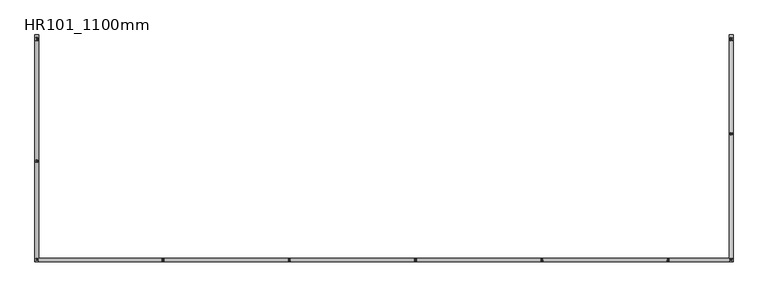
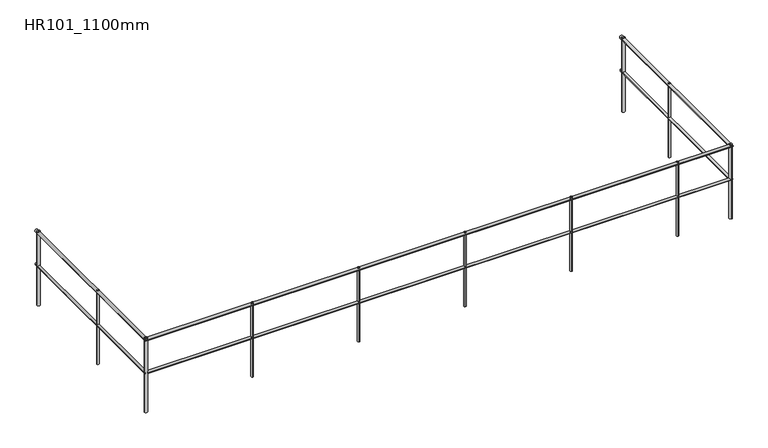
"""IFC4 building model written with IfcOpenShell, lengths in millimetres: railing geometry, HR101_1100mm."""

from ifc_helpers import new_model, si_unit, point, frame, frame_2d, origin, place, context, project, spatial, circle_curve, ellipse_curve, trimmed, segment, composite_curve, outline, extrude, source, transform, mapped, element, save
from ifc_brep_helpers import plane_surface, cylinder_surface, advanced_brep


def hr101_1100mm_fbcf2329(model_context):
    return source(origin(), model_context, "Body", "SolidModel", [
        advanced_brep(
        [(3942.0, 20699.5208589, 10633.005241), (3908.0, 20699.5208589, 10633.005241), (3942.0, 18041.5208589, 10633.005241), (3908.0, 18007.5208589, 10633.005241), (12158.0, 18041.5208589, 10633.005241), (12192.0, 18007.5208589, 10633.005241), (12158.0, 20699.5208589, 10633.005241), (12192.0, 20699.5208589, 10633.005241)],
        [
            (0, 1, circle_curve(frame((3925.0, 20699.5208589, 10633.005241), z_axis=(0.0, 1.0, 0.0), x_axis=(-1.0, 0.0, 0.0)), 17.0)),
            (1, 0, circle_curve(frame((3925.0, 20699.5208589, 10633.005241), z_axis=(0.0, 1.0, 0.0), x_axis=(-1.0, 0.0, 0.0)), 17.0)),
            (0, 2),
            (2, 3, ellipse_curve(frame((3925.0, 18024.5208589, 10633.005241), z_axis=(-0.7071067811865475, 0.7071067811865475, 0.0), x_axis=(0.7071067811865474, 0.7071067811865476, 0.0)), 24.0416306, 17.0)),
            (3, 1),
            (3, 2, ellipse_curve(frame((3925.0, 18024.5208589, 10633.005241), z_axis=(-0.7071067811865475, 0.7071067811865475, 0.0), x_axis=(0.7071067811865474, 0.7071067811865476, 0.0)), 24.0416306, 17.0)),
            (2, 4),
            (4, 5, ellipse_curve(frame((12175.0, 18024.5208589, 10633.005241), z_axis=(-0.7071067811865475, -0.7071067811865475, 0.0), x_axis=(-0.7071067811865476, 0.7071067811865474, 0.0)), 24.0416306, 17.0)),
            (5, 3),
            (5, 4, ellipse_curve(frame((12175.0, 18024.5208589, 10633.005241), z_axis=(-0.7071067811865475, -0.7071067811865475, 0.0), x_axis=(-0.7071067811865476, 0.7071067811865474, 0.0)), 24.0416306, 17.0)),
            (6, 7, circle_curve(frame((12175.0, 20699.5208589, 10633.005241), z_axis=(0.0, 1.0, 0.0), x_axis=(1.0, 0.0, 0.0)), 17.0)),
            (7, 6, circle_curve(frame((12175.0, 20699.5208589, 10633.005241), z_axis=(0.0, 1.0, 0.0), x_axis=(1.0, 0.0, 0.0)), 17.0)),
            (4, 6),
            (7, 5),
        ],
        [
            plane_surface(frame((3925.0, 20699.5208589, 10650.005241), z_axis=(0.0, 1.0, 0.0), x_axis=(0.0, 0.0, -1.0))),
            cylinder_surface(frame((3925.0, 20699.5208589, 10633.005241), z_axis=(0.0, 1.0, 0.0), x_axis=(-1.0, 0.0, 0.0)), 17.0),
            cylinder_surface(frame((3925.0, 18024.5208589, 10633.005241), z_axis=(-1.0, 0.0, 0.0), x_axis=(0.0, -1.0, 0.0)), 17.0),
            plane_surface(frame((12175.0, 20699.5208589, 10650.005241), z_axis=(0.0, 1.0, 0.0), x_axis=(0.0, 0.0, 1.0))),
            cylinder_surface(frame((12175.0, 18024.5208589, 10633.005241), z_axis=(0.0, -1.0, 0.0), x_axis=(1.0, 0.0, 0.0)), 17.0),
        ],
        [
            (0, [[1, 2]]),
            (1, [[-1, 3, 4, 5]]),
            (1, [[-2, -5, 6, -3]]),
            (2, [[-4, 7, 8, 9]]),
            (2, [[-6, -9, 10, -7]]),
            (3, [[11, 12]]),
            (4, [[-8, 13, -12, 14]]),
            (4, [[-10, -14, -11, -13]]),
        ],
    ),
        advanced_brep(
        [(3946.35, 20699.5208589, 11128.655241), (3903.65, 20699.5208589, 11128.655241), (3946.35, 18045.8708589, 11128.655241), (3903.65, 18003.1708589, 11128.655241), (12153.65, 18045.8708589, 11128.655241), (12196.35, 18003.1708589, 11128.655241), (12153.65, 20699.5208589, 11128.655241), (12196.35, 20699.5208589, 11128.655241)],
        [
            (0, 1, circle_curve(frame((3925.0, 20699.5208589, 11128.655241), z_axis=(0.0, 1.0, 0.0), x_axis=(-1.0, 0.0, 0.0)), 21.35)),
            (1, 0, circle_curve(frame((3925.0, 20699.5208589, 11128.655241), z_axis=(0.0, 1.0, 0.0), x_axis=(-1.0, 0.0, 0.0)), 21.35)),
            (0, 2),
            (2, 3, ellipse_curve(frame((3925.0, 18024.5208589, 11128.655241), z_axis=(-0.7071067811865475, 0.7071067811865475, 0.0), x_axis=(0.7071067811865474, 0.7071067811865476, 0.0)), 30.1934596, 21.35)),
            (3, 1),
            (3, 2, ellipse_curve(frame((3925.0, 18024.5208589, 11128.655241), z_axis=(-0.7071067811865475, 0.7071067811865475, 0.0), x_axis=(0.7071067811865474, 0.7071067811865476, 0.0)), 30.1934596, 21.35)),
            (2, 4),
            (4, 5, ellipse_curve(frame((12175.0, 18024.5208589, 11128.655241), z_axis=(-0.7071067811865475, -0.7071067811865475, 0.0), x_axis=(-0.7071067811865476, 0.7071067811865474, 0.0)), 30.1934596, 21.35)),
            (5, 3),
            (5, 4, ellipse_curve(frame((12175.0, 18024.5208589, 11128.655241), z_axis=(-0.7071067811865475, -0.7071067811865475, 0.0), x_axis=(-0.7071067811865476, 0.7071067811865474, 0.0)), 30.1934596, 21.35)),
            (6, 7, circle_curve(frame((12175.0, 20699.5208589, 11128.655241), z_axis=(0.0, 1.0, 0.0), x_axis=(1.0, 0.0, 0.0)), 21.35)),
            (7, 6, circle_curve(frame((12175.0, 20699.5208589, 11128.655241), z_axis=(0.0, 1.0, 0.0), x_axis=(1.0, 0.0, 0.0)), 21.35)),
            (4, 6),
            (7, 5),
        ],
        [
            plane_surface(frame((3925.0, 20699.5208589, 11150.005241), z_axis=(0.0, 1.0, 0.0), x_axis=(0.0, 0.0, -1.0))),
            cylinder_surface(frame((3925.0, 20699.5208589, 11128.655241), z_axis=(0.0, 1.0, 0.0), x_axis=(-1.0, 0.0, 0.0)), 21.35),
            cylinder_surface(frame((3925.0, 18024.5208589, 11128.655241), z_axis=(-1.0, 0.0, 0.0), x_axis=(0.0, -1.0, 0.0)), 21.35),
            plane_surface(frame((12175.0, 20699.5208589, 11150.005241), z_axis=(0.0, 1.0, 0.0), x_axis=(0.0, 0.0, 1.0))),
            cylinder_surface(frame((12175.0, 18024.5208589, 11128.655241), z_axis=(0.0, -1.0, 0.0), x_axis=(1.0, 0.0, 0.0)), 21.35),
        ],
        [
            (0, [[1, 2]]),
            (1, [[-1, 3, 4, 5]]),
            (1, [[-2, -5, 6, -3]]),
            (2, [[-4, 7, 8, 9]]),
            (2, [[-6, -9, 10, -7]]),
            (3, [[11, 12]]),
            (4, [[-8, 13, -12, 14]]),
            (4, [[-10, -14, -11, -13]]),
        ],
    ),
        extrude(outline(composite_curve([segment(trimmed(circle_curve(frame_2d((12175.0, 19524.5208589)), 15.0), [point((12190.0, 19524.5208589))], [point((12160.0, 19524.5208589))], False, "CARTESIAN"), True, "CONTINUOUS"), segment(trimmed(circle_curve(frame_2d((12175.0, 19524.5208589)), 15.0), [point((12160.0, 19524.5208589))], [point((12190.0, 19524.5208589))], False, "CARTESIAN"), True, "CONTINUOUS")], self_intersect=False)), frame((0.0, 0.0, 10050.005241), z_axis=(0.0, 0.0, 1.0), x_axis=(1.0, 0.0, 0.0)), (0.0, 0.0, 1.0), 1100.0),
        extrude(outline(composite_curve([segment(trimmed(circle_curve(frame_2d((11425.0, 18024.5208589)), 15.0), [point((11425.0, 18009.5208589))], [point((11425.0, 18039.5208589))], False, "CARTESIAN"), True, "CONTINUOUS"), segment(trimmed(circle_curve(frame_2d((11425.0, 18024.5208589)), 15.0), [point((11425.0, 18039.5208589))], [point((11425.0, 18009.5208589))], False, "CARTESIAN"), True, "CONTINUOUS")], self_intersect=False)), frame((0.0, 0.0, 10050.005241), z_axis=(0.0, 0.0, 1.0), x_axis=(1.0, 0.0, 0.0)), (0.0, 0.0, 1.0), 1100.0),
        extrude(outline(composite_curve([segment(trimmed(circle_curve(frame_2d((9925.0, 18024.5208589)), 15.0), [point((9925.0, 18009.5208589))], [point((9925.0, 18039.5208589))], False, "CARTESIAN"), True, "CONTINUOUS"), segment(trimmed(circle_curve(frame_2d((9925.0, 18024.5208589)), 15.0), [point((9925.0, 18039.5208589))], [point((9925.0, 18009.5208589))], False, "CARTESIAN"), True, "CONTINUOUS")], self_intersect=False)), frame((0.0, 0.0, 10050.005241), z_axis=(0.0, 0.0, 1.0), x_axis=(1.0, 0.0, 0.0)), (0.0, 0.0, 1.0), 1100.0),
        extrude(outline(composite_curve([segment(trimmed(circle_curve(frame_2d((8425.0, 18024.5208589)), 15.0), [point((8425.0, 18009.5208589))], [point((8425.0, 18039.5208589))], False, "CARTESIAN"), True, "CONTINUOUS"), segment(trimmed(circle_curve(frame_2d((8425.0, 18024.5208589)), 15.0), [point((8425.0, 18039.5208589))], [point((8425.0, 18009.5208589))], False, "CARTESIAN"), True, "CONTINUOUS")], self_intersect=False)), frame((0.0, 0.0, 10050.005241), z_axis=(0.0, 0.0, 1.0), x_axis=(1.0, 0.0, 0.0)), (0.0, 0.0, 1.0), 1100.0),
        extrude(outline(composite_curve([segment(trimmed(circle_curve(frame_2d((6925.0, 18024.5208589)), 15.0), [point((6925.0, 18009.5208589))], [point((6925.0, 18039.5208589))], False, "CARTESIAN"), True, "CONTINUOUS"), segment(trimmed(circle_curve(frame_2d((6925.0, 18024.5208589)), 15.0), [point((6925.0, 18039.5208589))], [point((6925.0, 18009.5208589))], False, "CARTESIAN"), True, "CONTINUOUS")], self_intersect=False)), frame((0.0, 0.0, 10050.005241), z_axis=(0.0, 0.0, 1.0), x_axis=(1.0, 0.0, 0.0)), (0.0, 0.0, 1.0), 1100.0),
        extrude(outline(composite_curve([segment(trimmed(circle_curve(frame_2d((5425.0, 18024.5208589)), 15.0), [point((5425.0, 18009.5208589))], [point((5425.0, 18039.5208589))], False, "CARTESIAN"), True, "CONTINUOUS"), segment(trimmed(circle_curve(frame_2d((5425.0, 18024.5208589)), 15.0), [point((5425.0, 18039.5208589))], [point((5425.0, 18009.5208589))], False, "CARTESIAN"), True, "CONTINUOUS")], self_intersect=False)), frame((0.0, 0.0, 10050.005241), z_axis=(0.0, 0.0, 1.0), x_axis=(1.0, 0.0, 0.0)), (0.0, 0.0, 1.0), 1100.0),
        extrude(outline(composite_curve([segment(trimmed(circle_curve(frame_2d((3925.0, 19199.5208589)), 15.0), [point((3910.0, 19199.5208589))], [point((3940.0, 19199.5208589))], False, "CARTESIAN"), True, "CONTINUOUS"), segment(trimmed(circle_curve(frame_2d((3925.0, 19199.5208589)), 15.0), [point((3940.0, 19199.5208589))], [point((3910.0, 19199.5208589))], False, "CARTESIAN"), True, "CONTINUOUS")], self_intersect=False)), frame((0.0, 0.0, 10050.005241), z_axis=(0.0, 0.0, 1.0), x_axis=(1.0, 0.0, 0.0)), (0.0, 0.0, 1.0), 1100.0),
        extrude(outline(composite_curve([segment(trimmed(circle_curve(frame_2d((12175.0, 18024.5208589)), 21.35), [point((12175.0, 18003.1708589))], [point((12175.0, 18045.8708589))], False, "CARTESIAN"), True, "CONTINUOUS"), segment(trimmed(circle_curve(frame_2d((12175.0, 18024.5208589)), 21.35), [point((12175.0, 18045.8708589))], [point((12175.0, 18003.1708589))], False, "CARTESIAN"), True, "CONTINUOUS")], self_intersect=False)), frame((0.0, 0.0, 10050.005241), z_axis=(0.0, 0.0, 1.0), x_axis=(1.0, 0.0, 0.0)), (0.0, 0.0, 1.0), 1100.0),
        extrude(outline(composite_curve([segment(trimmed(circle_curve(frame_2d((3925.0, 18024.5208589)), 21.35), [point((3903.65, 18024.5208589))], [point((3946.35, 18024.5208589))], False, "CARTESIAN"), True, "CONTINUOUS"), segment(trimmed(circle_curve(frame_2d((3925.0, 18024.5208589)), 21.35), [point((3946.35, 18024.5208589))], [point((3903.65, 18024.5208589))], False, "CARTESIAN"), True, "CONTINUOUS")], self_intersect=False)), frame((0.0, 0.0, 10050.005241), z_axis=(0.0, 0.0, 1.0), x_axis=(1.0, 0.0, 0.0)), (0.0, 0.0, 1.0), 1100.0),
        extrude(outline(composite_curve([segment(trimmed(circle_curve(frame_2d((12175.0, 20649.5208589)), 21.35), [point((12196.35, 20649.5208589))], [point((12153.65, 20649.5208589))], False, "CARTESIAN"), True, "CONTINUOUS"), segment(trimmed(circle_curve(frame_2d((12175.0, 20649.5208589)), 21.35), [point((12153.65, 20649.5208589))], [point((12196.35, 20649.5208589))], False, "CARTESIAN"), True, "CONTINUOUS")], self_intersect=False)), frame((0.0, 0.0, 10050.005241), z_axis=(0.0, 0.0, 1.0), x_axis=(1.0, 0.0, 0.0)), (0.0, 0.0, 1.0), 1100.0),
        extrude(outline(composite_curve([segment(trimmed(circle_curve(frame_2d((3925.0, 20649.5208589)), 21.35), [point((3903.65, 20649.5208589))], [point((3946.35, 20649.5208589))], False, "CARTESIAN"), True, "CONTINUOUS"), segment(trimmed(circle_curve(frame_2d((3925.0, 20649.5208589)), 21.35), [point((3946.35, 20649.5208589))], [point((3903.65, 20649.5208589))], False, "CARTESIAN"), True, "CONTINUOUS")], self_intersect=False)), frame((0.0, 0.0, 10050.005241), z_axis=(0.0, 0.0, 1.0), x_axis=(1.0, 0.0, 0.0)), (0.0, 0.0, 1.0), 1100.0),
    ])


if __name__ == "__main__":
    model = new_model("IFC4")
    model_context = context("Model", 3, world=origin())
    ifc_project = project(units=[si_unit("LENGTHUNIT", "METRE", prefix="MILLI")], contexts=[model_context])
    site = spatial("IfcSite", under=ifc_project)
    building = spatial("IfcBuilding", under=site)
    placement = place(None, origin())
    hr101_1100mm_shape = hr101_1100mm_fbcf2329(model_context)
    element("IfcRailing", 1, ObjectType="HR101_1100mm", at=placement, inside=building, context=model_context, shape_type="MappedRepresentation", body=[
        mapped(hr101_1100mm_shape, transform((0.0, 0.0, 0.0), x_axis=(1.0, 0.0, 0.0), y_axis=(0.0, 1.0, 0.0), z_axis=(0.0, 0.0, 1.0))),
    ])
    save(model, "model.ifc")

# Revit data of these elements
# Element 1 (IfcRailing, "HR101_1100mm")
#   Materials on its faces: "S02AA020-00001_Steel Handrails"
# Materials
#   "S02AA020-00001_Steel Handrails": class "Metal", colour RGB 148 148 148, transparency 0, Description = "STEEL HANDRAIL(TYP.)", Cost = 0
